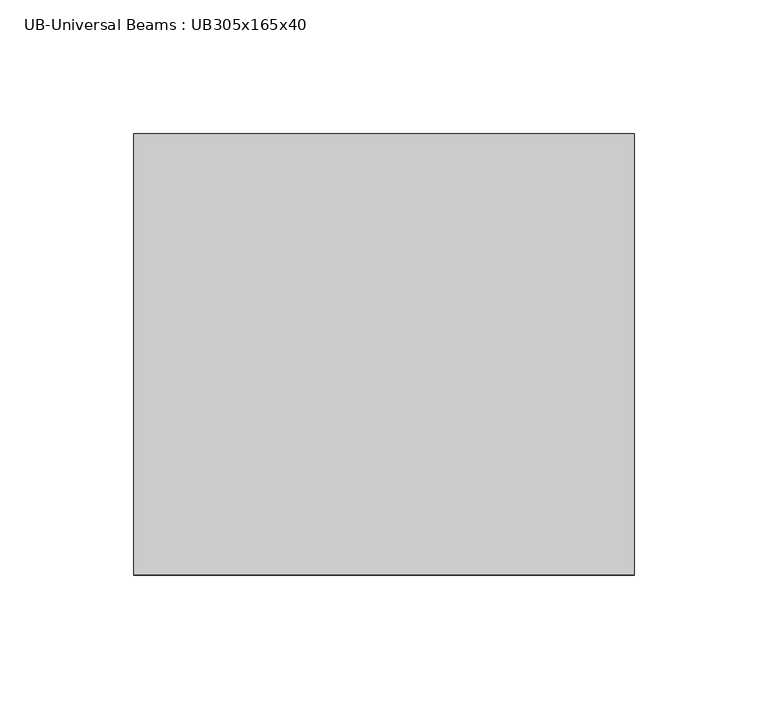
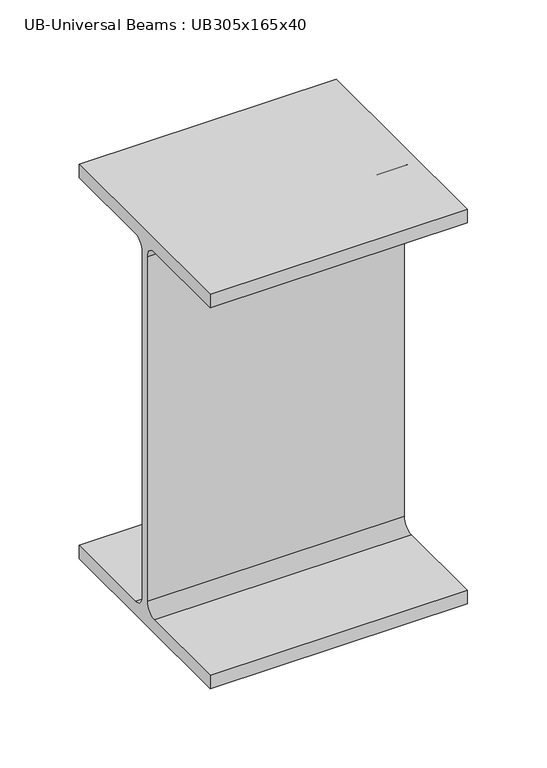
"""IFC4 building model written with IfcOpenShell, lengths in millimetres: beam geometry, UB-Universal Beams : UB305x165x40."""

import ifcopenshell
import ifcopenshell.guid

model = None  # the IFC model being written
_history = None  # IfcOwnerHistory: only IFC2X3 demands one
_inside = {}  # id of a spatial element -> (the spatial element, [elements in it])
_under = {}  # id of a project, library or spatial element -> (it, [spatial elements below it])
_declared = {}  # id of a project -> (the project, [libraries it declares])
_typed = {}  # id of a type object -> (the type object, [elements of that type])
_made_of = {}  # id of a material, layer set ... -> (it, [elements and type objects made of it])


def new_model(schema):
    """Start an empty IFC model of exactly this schema.

    Asked for "IFC4X3", IfcOpenShell would pick the latest addendum, in which some entities
    have other attributes; the version numbers below select the first issue.
    IFC2X3 requires an IfcOwnerHistory on every rooted entity: one is made here for all.
    """
    global model, _history
    if schema == "IFC4X3":
        model = ifcopenshell.file(schema_version=(4, 3, 0, 0))
    else:
        model = ifcopenshell.file(schema=schema)
    _inside.clear()
    _under.clear()
    _declared.clear()
    _typed.clear()
    _made_of.clear()
    _history = None
    if model.schema == "IFC2X3":
        org = make("IfcOrganization", Name="unknown")
        user = make(
            "IfcPersonAndOrganization",
            ThePerson=make("IfcPerson", FamilyName="unknown"),
            TheOrganization=org,
        )
        app = make(
            "IfcApplication",
            ApplicationDeveloper=org,
            Version="unknown",
            ApplicationFullName="unknown",
            ApplicationIdentifier="unknown",
        )
        _history = make(
            "IfcOwnerHistory",
            OwningUser=user,
            OwningApplication=app,
            ChangeAction="ADDED",
            CreationDate=0,
        )
    return model


def make(cls, **values):
    """One entity of the class cls with the attributes given. An attribute that is None is left unset."""
    return model.create_entity(
        cls, **{name: value for name, value in values.items() if value is not None}
    )


def rooted(cls, **values):
    """An entity with a GlobalId (a new one), such as an element, a storey or a relation."""
    return make(cls, GlobalId=ifcopenshell.guid.new(), OwnerHistory=_history, **values)


def si_unit(unit_type, name, prefix=None):
    """IfcSIUnit, for example si_unit("LENGTHUNIT", "METRE", prefix="MILLI")."""
    return make("IfcSIUnit", UnitType=unit_type, Prefix=prefix, Name=name)


def assignment(units):
    """IfcUnitAssignment: the units of a project."""
    return None if units is None else make("IfcUnitAssignment", Units=units)


def point(xyz):
    """IfcCartesianPoint."""
    return None if xyz is None else make("IfcCartesianPoint", Coordinates=xyz)


def direction(xyz):
    """IfcDirection."""
    return None if xyz is None else make("IfcDirection", DirectionRatios=xyz)


def frame(location, z_axis=None, x_axis=None):
    """IfcAxis2Placement3D, a coordinate frame: its origin and axes. An axis left out is left unset."""
    return make(
        "IfcAxis2Placement3D",
        Location=point(location),
        Axis=direction(z_axis),
        RefDirection=direction(x_axis),
    )


def frame_2d(location, x_axis=None):
    """IfcAxis2Placement2D, a coordinate frame in the plane: its origin and x axis."""
    return make(
        "IfcAxis2Placement2D", Location=point(location), RefDirection=direction(x_axis)
    )


def origin():
    """The frame at (0, 0, 0) with its axes left unset."""
    return frame((0.0, 0.0, 0.0))


def place(relative_to, where):
    """IfcLocalPlacement: puts the frame where relative to a parent placement (None: the world)."""
    return make(
        "IfcLocalPlacement", PlacementRelTo=relative_to, RelativePlacement=where
    )


def context(
    kind, dimensions, precision=None, world=None, true_north=None, identifier=None
):
    """IfcGeometricRepresentationContext, for example the 3D "Model" context."""
    return make(
        "IfcGeometricRepresentationContext",
        ContextIdentifier=identifier,
        ContextType=kind,
        CoordinateSpaceDimension=dimensions,
        Precision=precision,
        WorldCoordinateSystem=world,
        TrueNorth=true_north,
    )


def project(units=None, contexts=None):
    """IfcProject with its units and contexts."""
    return rooted(
        "IfcProject",
        Name="project",
        RepresentationContexts=contexts,
        UnitsInContext=assignment(units),
    )


def spatial(cls, under=None, at=None, **own):
    """A site, building, storey or space (cls), placed at a placement, below another one or the project."""
    s = rooted(cls, ObjectPlacement=at, **own)
    if under is not None:
        _under.setdefault(under.id(), (under, []))[1].append(s)
    return s


def polyline(points):
    """IfcPolyline through the points."""
    return make("IfcPolyline", Points=[point(p) for p in points])


def circle_curve(where, radius):
    """IfcCircle in the frame where."""
    return make("IfcCircle", Position=where, Radius=radius)


def trimmed(basis, trim1, trim2, sense, master):
    """IfcTrimmedCurve: the piece of a basis curve between two trims."""
    return make(
        "IfcTrimmedCurve",
        BasisCurve=basis,
        Trim1=trim1,
        Trim2=trim2,
        SenseAgreement=sense,
        MasterRepresentation=master,
    )


def segment(curve, same_sense, transition):
    """IfcCompositeCurveSegment."""
    return make(
        "IfcCompositeCurveSegment",
        Transition=transition,
        SameSense=same_sense,
        ParentCurve=curve,
    )


def composite_curve(segments, self_intersect=None):
    """IfcCompositeCurve: segments joined end to end."""
    return make("IfcCompositeCurve", Segments=segments, SelfIntersect=self_intersect)


def outline(outer, holes=None, kind="AREA"):
    """IfcArbitraryClosedProfileDef: a profile drawn as a closed curve; with holes, ...WithVoids."""
    if holes is None:
        return make("IfcArbitraryClosedProfileDef", ProfileType=kind, OuterCurve=outer)
    return make(
        "IfcArbitraryProfileDefWithVoids",
        ProfileType=kind,
        OuterCurve=outer,
        InnerCurves=holes,
    )


def extrude(swept, where, along, depth):
    """IfcExtrudedAreaSolid: the profile swept, set in the frame where, extruded along a direction by depth."""
    return make(
        "IfcExtrudedAreaSolid",
        SweptArea=swept,
        Position=where,
        ExtrudedDirection=direction(along),
        Depth=depth,
    )


def shape(context_of_items, identifier, shape_type, items):
    """IfcShapeRepresentation: the items that make up one representation, for example the "Body"."""
    return make(
        "IfcShapeRepresentation",
        ContextOfItems=context_of_items,
        RepresentationIdentifier=identifier,
        RepresentationType=shape_type,
        Items=items,
    )


def source(mapping_origin, context_of_items, identifier, shape_type, items):
    """IfcRepresentationMap: a shape defined once, which mapped items show again and again."""
    return make(
        "IfcRepresentationMap",
        MappingOrigin=mapping_origin,
        MappedRepresentation=shape(context_of_items, identifier, shape_type, items),
    )


def transform(
    local_origin,
    x_axis=None,
    y_axis=None,
    z_axis=None,
    scale=None,
    scale2=None,
    scale3=None,
    uniform=True,
):
    """IfcCartesianTransformationOperator3D, or its non-uniform kind. x_axis, y_axis, z_axis: its Axis1, 2, 3."""
    if uniform:
        return make(
            "IfcCartesianTransformationOperator3D",
            Axis1=direction(x_axis),
            Axis2=direction(y_axis),
            LocalOrigin=point(local_origin),
            Scale=scale,
            Axis3=direction(z_axis),
        )
    return make(
        "IfcCartesianTransformationOperator3DnonUniform",
        Axis1=direction(x_axis),
        Axis2=direction(y_axis),
        LocalOrigin=point(local_origin),
        Scale=scale,
        Axis3=direction(z_axis),
        Scale2=scale2,
        Scale3=scale3,
    )


def mapped(mapping_source, mapping_target):
    """IfcMappedItem: shows the shape of a source again, moved by a transform."""
    return make(
        "IfcMappedItem", MappingSource=mapping_source, MappingTarget=mapping_target
    )


def made_of(thing, what):
    """Note that an element or type object is made of a material, layer set ...; save() writes the relation."""
    if what is not None:
        _made_of.setdefault(what.id(), (what, []))[1].append(thing)
    return thing


def element(
    cls,
    number,
    at=None,
    inside=None,
    cuts=None,
    type_object=None,
    material=None,
    context=None,
    identifier="Body",
    shape_type=None,
    held_by="IfcProductDefinitionShape",
    body=None,
    shapes=None,
    **own,
):
    """One element of the class cls, such as IfcWall. Its Tag is "e" and its number.

    at: its placement. inside: the storey or other place that contains it. cuts: it is an
    opening in that element (IfcRelVoidsElement). A single representation is given by context,
    identifier, shape_type and body (its items); several are given by shapes. held_by: the class
    of the entity that holds the representations. save() writes the other relations.
    """
    e = rooted(cls, Tag="e%d" % number, ObjectPlacement=at, **own)
    if body is not None:
        shapes = [shape(context, identifier, shape_type, body)]
    if shapes is not None:
        e.Representation = make(held_by, Representations=shapes)
    if inside is not None:
        _inside.setdefault(inside.id(), (inside, []))[1].append(e)
    if cuts is not None:
        rooted(
            "IfcRelVoidsElement", RelatingBuildingElement=cuts, RelatedOpeningElement=e
        )
    if type_object is not None:
        _typed.setdefault(type_object.id(), (type_object, []))[1].append(e)
    return made_of(e, material)


def aggregate(whole, parts):
    """IfcRelAggregates: a whole, such as a stair, and the parts it consists of."""
    return rooted("IfcRelAggregates", RelatingObject=whole, RelatedObjects=parts)


def save(model, path):
    """Write the relations noted so far, then the file.

    IfcRelAggregates (storeys below a building ...), IfcRelContainedInSpatialStructure (elements
    in a storey), IfcRelDefinesByType, IfcRelAssociatesMaterial and IfcRelDeclares: one each for
    every whole, place, type object, material and project.
    """
    for whole, parts in _under.values():
        aggregate(whole, parts)
    for where, things in _inside.values():
        rooted(
            "IfcRelContainedInSpatialStructure",
            RelatedElements=things,
            RelatingStructure=where,
        )
    for kind, things in _typed.values():
        rooted("IfcRelDefinesByType", RelatedObjects=things, RelatingType=kind)
    for what, things in _made_of.values():
        rooted("IfcRelAssociatesMaterial", RelatedObjects=things, RelatingMaterial=what)
    for by, libraries in _declared.values():
        rooted("IfcRelDeclares", RelatingContext=by, RelatedDefinitions=libraries)
    model.write(path)


def ub_universal_beams_ub305x165x40_16995a82(model_context):
    return source(origin(), model_context, "Body", "SweptSolid", [
        extrude(outline(composite_curve([segment(polyline([(82.5, -141.5), (82.5, -151.7), (-82.5, -151.7), (-82.5, -141.5), (-11.9, -141.5)]), True, "CONTINUOUS"), segment(trimmed(circle_curve(frame_2d((-11.9, -132.6)), 8.9), [point((-11.9, -141.5))], [point((-3.0, -132.6))], True, "CARTESIAN"), True, "CONTINUOUS"), segment(polyline([(-3.0, -132.6), (-3.0, 132.6)]), True, "CONTINUOUS"), segment(trimmed(circle_curve(frame_2d((-11.9, 132.6)), 8.9), [point((-3.0, 132.6))], [point((-11.9, 141.5))], True, "CARTESIAN"), True, "CONTINUOUS"), segment(polyline([(-11.9, 141.5), (-82.5, 141.5), (-82.5, 151.7), (82.5, 151.7), (82.5, 141.5), (11.9, 141.5)]), True, "CONTINUOUS"), segment(trimmed(circle_curve(frame_2d((11.9, 132.6)), 8.9), [point((11.9, 141.5))], [point((3.0, 132.6))], True, "CARTESIAN"), True, "CONTINUOUS"), segment(polyline([(3.0, 132.6), (3.0, -132.6)]), True, "CONTINUOUS"), segment(trimmed(circle_curve(frame_2d((11.9, -132.6)), 8.9), [point((3.0, -132.6))], [point((11.9, -141.5))], True, "CARTESIAN"), True, "CONTINUOUS"), segment(polyline([(11.9, -141.5), (82.5, -141.5)]), True, "CONTINUOUS")], self_intersect=False)), frame((-87.2, 0.0, 0.0), z_axis=(1.0, 0.0, 0.0), x_axis=(0.0, 1.0, 0.0)), (0.0, 0.0, 1.0), 187.2),
    ])


if __name__ == "__main__":
    model = new_model("IFC4")
    model_context = context("Model", 3, world=origin())
    ifc_project = project(units=[si_unit("LENGTHUNIT", "METRE", prefix="MILLI")], contexts=[model_context])
    site = spatial("IfcSite", under=ifc_project)
    building = spatial("IfcBuilding", under=site)
    placement = place(None, origin())
    ub_universal_beams_ub305x165x40_shape = ub_universal_beams_ub305x165x40_16995a82(model_context)
    element("IfcBeam", 1, ObjectType="UB-Universal Beams : UB305x165x40", at=placement, inside=building, context=model_context, shape_type="MappedRepresentation", body=[
        mapped(ub_universal_beams_ub305x165x40_shape, transform((0.0, 0.0, 0.0), x_axis=(1.0, 0.0, 0.0), y_axis=(0.0, 1.0, 0.0), z_axis=(0.0, 0.0, 1.0))),
    ])
    save(model, "model.ifc")

# Revit data of these elements
# Type "UB-Universal Beams : UB305x165x40"
#   Section Name Key = "UB305X165X40"
#   Width = 16.5 cm
#   Web Thickness = 0.6 cm
#   Web Fillet = 0.89 cm
#   Warping Constant = 164000.0 cm⁶
#   Torsional Moment of Inertia = 14.70 cm⁴
#   Section Area = 51.3 cm²
#   Plastic Modulus weak axis = 142.0 cm³
#   Plastic Modulus strong axis = 623.0 cm³
#   Nominal Weight = 40.2999 kgf/m
#   Moment of Inertia weak axis = 764.00 cm⁴
#   Moment of Inertia strong axis = 8503.00 cm⁴
#   Height = 30.34 cm
#   Flange Thickness = 1.02 cm
#   Elastic Modulus weak axis = 92.6 cm³
#   Elastic Modulus strong axis = 560.0 cm³
#   Centroid Vertical = 15.17 cm
#   Centroid Horizontal = 8.25 cm
#   Bolt Spacing = 9.0 cm
#   Length [instance default] = 1500 mm
#   Structural Material [instance default] = Metal - Steel 43-275
#   Type Comments = ""
#   Assembly Code = ""
# Element 1 (IfcBeam, "UB-Universal Beams : UB305x165x40")
#   Materials on its faces: "Metal - Steel 43-275"
# Materials
#   "Metal - Steel 43-275": class "Metal", colour RGB 247 247 247, transparency 0, Cost = 0
